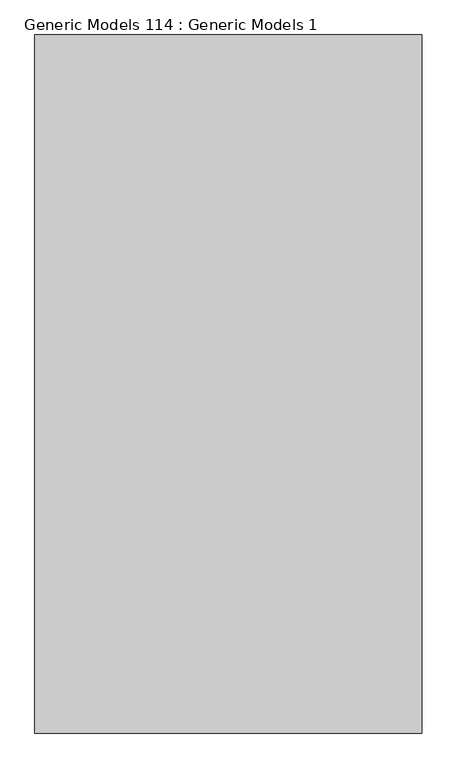
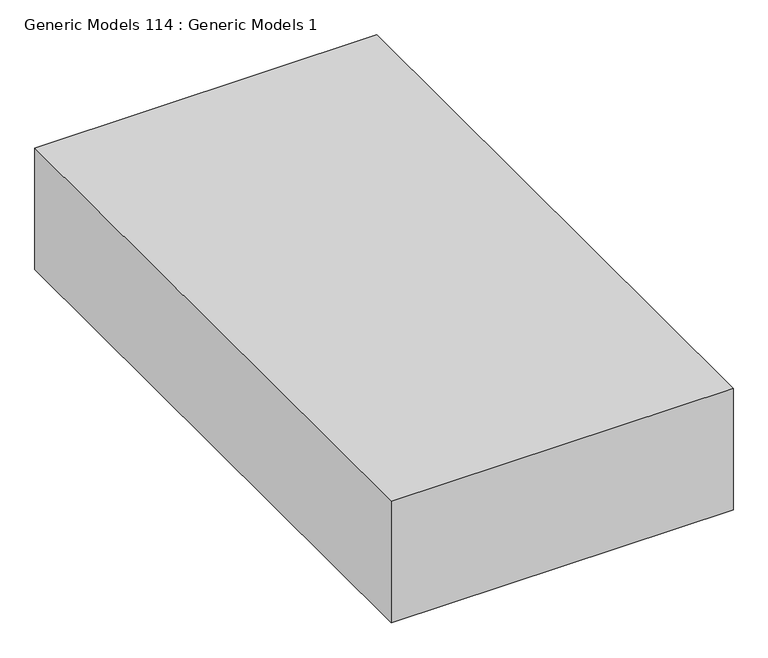
"""IFC4 building model written with IfcOpenShell, lengths in millimetres: proxy geometry, Generic Models 114 : Generic Models 1."""

from ifc_helpers import new_model, si_unit, frame, origin, place, context, project, spatial, polyline, outline, extrude, source, transform, mapped, element, save


def generic_models_114_generic_models_1_a6fb1c2c(model_context):
    return source(origin(), model_context, "Body", "SweptSolid", [
        extrude(outline(polyline([(51642.1451407, 1219.2), (51642.1451407, 0.0), (50965.9242022, 0.0), (50965.9242022, 1219.2), (51642.1451407, 1219.2)])), frame((0.0, 0.0, 5237.6235034), z_axis=(0.0, 0.0, 1.0), x_axis=(1.0, 0.0, 0.0)), (0.0, 0.0, 1.0), 254.0),
    ])


if __name__ == "__main__":
    model = new_model("IFC4")
    model_context = context("Model", 3, world=origin())
    ifc_project = project(units=[si_unit("LENGTHUNIT", "METRE", prefix="MILLI")], contexts=[model_context])
    site = spatial("IfcSite", under=ifc_project)
    building = spatial("IfcBuilding", under=site)
    placement = place(None, origin())
    generic_models_114_generic_models_1_shape = generic_models_114_generic_models_1_a6fb1c2c(model_context)
    element("IfcBuildingElementProxy", 1, Name="Generic Models 114 : Generic Models 1", ObjectType="Generic Models 114 : Generic Models 1", at=placement, inside=building, context=model_context, shape_type="MappedRepresentation", body=[
        mapped(generic_models_114_generic_models_1_shape, transform((0.0, 0.0, 0.0), x_axis=(1.0, 0.0, 0.0), y_axis=(0.0, 1.0, 0.0), z_axis=(0.0, 0.0, 1.0))),
    ])
    save(model, "model.ifc")

# Revit data of these elements
# Element 1 (IfcBuildingElementProxy, "Generic Models 114 : Generic Models 1")
#   Materials on its faces: "SOUND BATT. INSULATION"
# Materials
#   "SOUND BATT. INSULATION": class "Unassigned", colour RGB 255 255 255, transparency 0, Cost = 0
